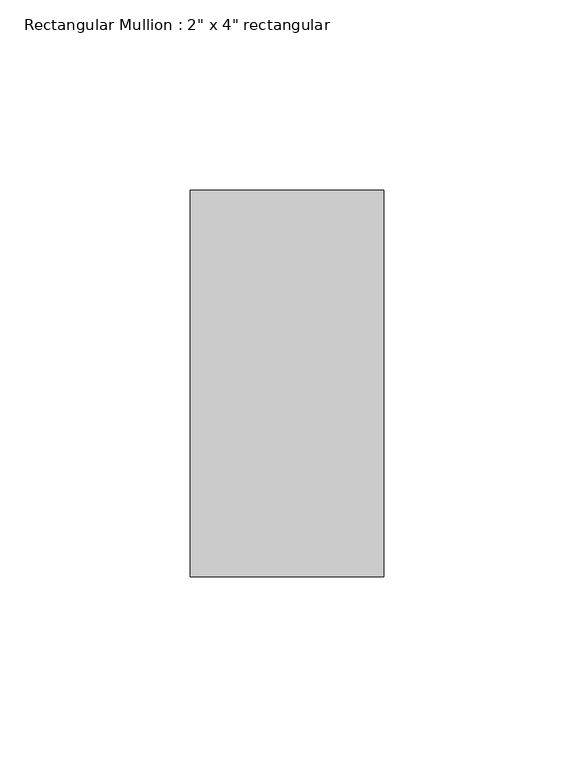
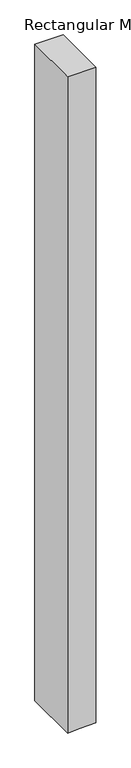
"""IFC4 building model written with IfcOpenShell, lengths in millimetres: member geometry."""

from ifc_helpers import new_model, si_unit, frame, origin, place, context, project, spatial, polyline, outline, extrude, source, transform, mapped, element, save


def member_65ffc098(model_context):
    return source(origin(), model_context, "Body", "SweptSolid", [
        extrude(outline(polyline([(0.0, 25.4), (0.0, -25.4), (-1248.1755325, -25.4), (-1247.2053172, -2.1148317), (-1246.0588658, 25.4), (0.0, 25.4)])), frame((0.0, -50.8, 0.0), z_axis=(0.0, 1.0, 0.0), x_axis=(0.0, 0.0, 1.0)), (0.0, 0.0, 1.0), 101.6),
    ])


if __name__ == "__main__":
    model = new_model("IFC4")
    model_context = context("Model", 3, world=origin())
    ifc_project = project(units=[si_unit("LENGTHUNIT", "METRE", prefix="MILLI")], contexts=[model_context])
    site = spatial("IfcSite", under=ifc_project)
    building = spatial("IfcBuilding", under=site)
    placement = place(None, origin())
    member_shape = member_65ffc098(model_context)
    element("IfcMember", 1, ObjectType="Rectangular Mullion : 2\" x 4\" rectangular", at=placement, inside=building, context=model_context, shape_type="MappedRepresentation", body=[
        mapped(member_shape, transform((0.0, 0.0, 0.0), x_axis=(1.0, 0.0, 0.0), y_axis=(0.0, 1.0, 0.0), z_axis=(0.0, 0.0, 1.0))),
    ])
    save(model, "model.ifc")

# Revit data of these elements
# Type "Rectangular Mullion : 2\" x 4\" rectangular"
#   built-in parameter 1007304 = 0.333333 (stored number, unit not read)
#   built-in parameter 1007301 = 0.0833333 (stored number, unit not read)
#   built-in parameter 1007300 = 0.0833333 (stored number, unit not read)
# Element 1 (IfcMember, "Rectangular Mullion : 2\" x 4\" rectangular")
#   Materials on its faces: "PAINTED STEEL C CHANNEL"
# Materials
#   "PAINTED STEEL C CHANNEL": class "Generic", colour RGB 88 62 61, transparency 0, Cost = 0
